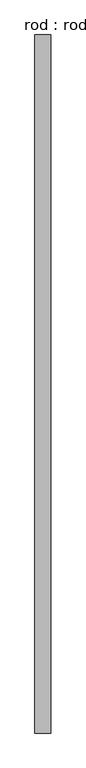
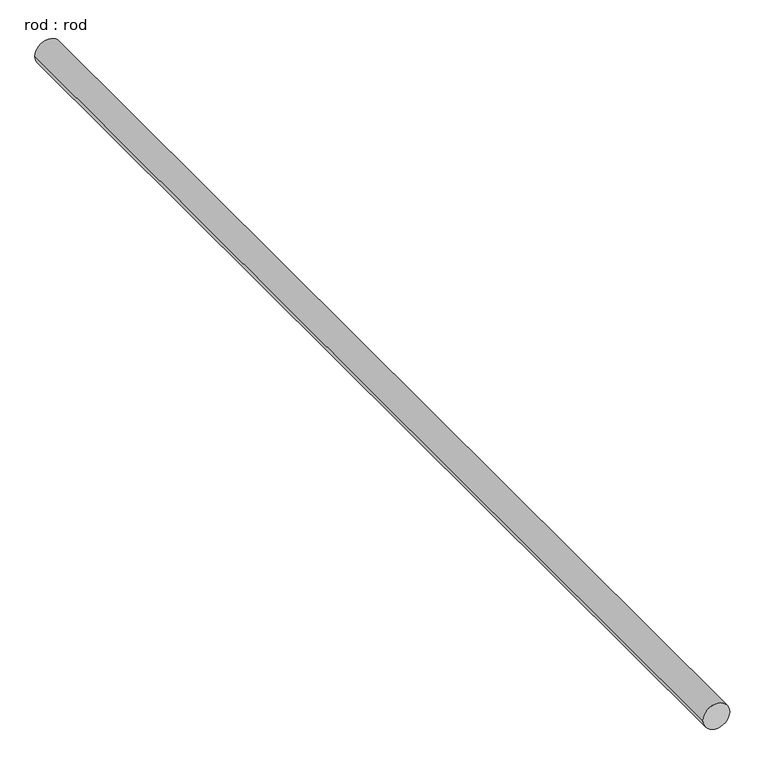
"""IFC4 building model written with IfcOpenShell, lengths in millimetres: proxy geometry, rod : rod."""

from ifc_helpers import new_model, si_unit, point, frame, frame_2d, origin, place, context, project, spatial, circle_curve, trimmed, segment, composite_curve, outline, extrude, source, transform, mapped, element, save


def rod_rod_4dd52836(model_context):
    return source(origin(), model_context, "Body", "SweptSolid", [
        extrude(outline(composite_curve([segment(trimmed(circle_curve(frame_2d((0.0108462, 0.0)), 200.0), [point((0.0108462, 200.0))], [point((0.0108462, -200.0))], False, "CARTESIAN"), True, "CONTINUOUS"), segment(trimmed(circle_curve(frame_2d((0.0108462, 0.0)), 200.0), [point((0.0108462, -200.0))], [point((0.0108462, 200.0))], False, "CARTESIAN"), True, "CONTINUOUS")], self_intersect=False)), frame((0.0, -4612.8291561, 0.0), z_axis=(0.0, 1.0, 0.0), x_axis=(0.0, 0.0, 1.0)), (0.0, 0.0, 1.0), 17411.1155428),
    ])


if __name__ == "__main__":
    model = new_model("IFC4")
    model_context = context("Model", 3, world=origin())
    ifc_project = project(units=[si_unit("LENGTHUNIT", "METRE", prefix="MILLI")], contexts=[model_context])
    site = spatial("IfcSite", under=ifc_project)
    building = spatial("IfcBuilding", under=site)
    placement = place(None, origin())
    rod_rod_shape = rod_rod_4dd52836(model_context)
    element("IfcBuildingElementProxy", 1, Name="rod : rod", ObjectType="rod : rod", at=placement, inside=building, context=model_context, shape_type="MappedRepresentation", body=[
        mapped(rod_rod_shape, transform((0.0, 0.0, 0.0), x_axis=(1.0, 0.0, 0.0), y_axis=(0.0, 1.0, 0.0), z_axis=(0.0, 0.0, 1.0))),
    ])
    save(model, "model.ifc")

# Revit data of these elements
# Type "rod : rod"
#   Default Elevation = 0
